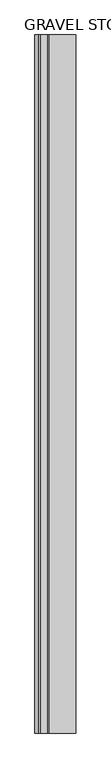
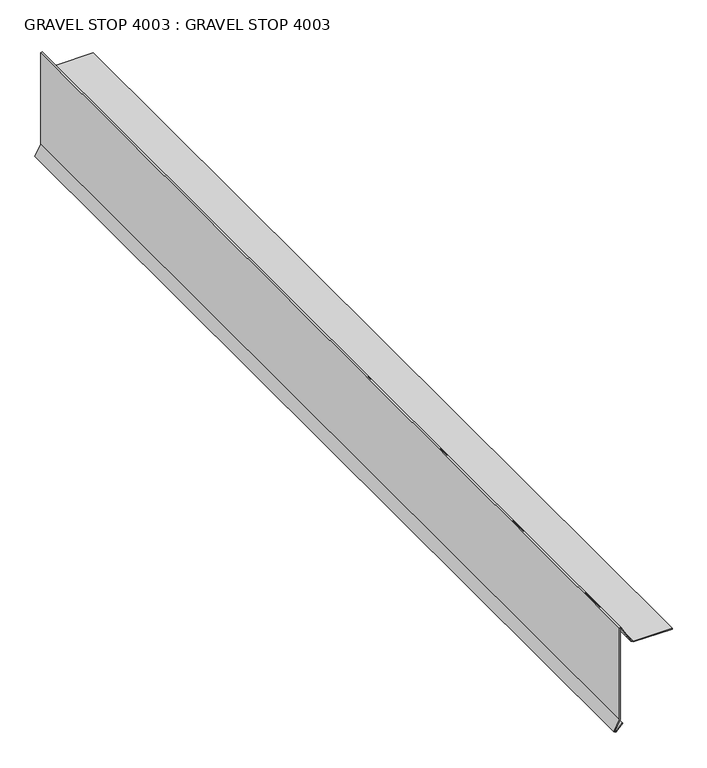
"""IFC4 building model written with IfcOpenShell, lengths in millimetres: proxy geometry, GRAVEL STOP 4003 : GRAVEL STOP 4003."""

from ifc_helpers import new_model, si_unit, frame, origin, place, context, project, spatial, polyline, outline, extrude, source, transform, mapped, element, save


def gravel_stop_4003_gravel_stop_4003_885a835c(model_context):
    return source(origin(), model_context, "Body", "SweptSolid", [
        extrude(outline(polyline([(40077.410403, -2814.9855343), (40091.8049, -2800.5910374), (40092.8027062, -2801.5888435), (40079.2807815, -2815.1107682), (40080.9054201, -2817.2404183), (40101.495749, -2805.9993985), (40293.447969, -2805.9993985), (40293.699878, -2805.0592614), (40258.5078708, -2784.7411466), (40255.9633674, -2780.3339375), (40255.9633674, -2702.4979247), (40257.3744784, -2702.4979247), (40257.3744784, -2779.9558314), (40259.5408757, -2783.7081416), (40295.3431515, -2804.3785952), (40294.5307525, -2807.4105095), (40101.8558531, -2807.4105095), (40080.5182783, -2819.0594785), (40077.410403, -2814.9855343)])), frame((0.0, -1052.8906573, 0.0), z_axis=(0.0, 1.0, 0.0), x_axis=(0.0, 0.0, 1.0)), (0.0, 0.0, 1.0), 2000.25),
    ])


if __name__ == "__main__":
    model = new_model("IFC4")
    model_context = context("Model", 3, world=origin())
    ifc_project = project(units=[si_unit("LENGTHUNIT", "METRE", prefix="MILLI")], contexts=[model_context])
    site = spatial("IfcSite", under=ifc_project)
    building = spatial("IfcBuilding", under=site)
    placement = place(None, origin())
    gravel_stop_4003_gravel_stop_4003_shape = gravel_stop_4003_gravel_stop_4003_885a835c(model_context)
    element("IfcBuildingElementProxy", 1, Name="GRAVEL STOP 4003 : GRAVEL STOP 4003", ObjectType="GRAVEL STOP 4003 : GRAVEL STOP 4003", at=placement, inside=building, context=model_context, shape_type="MappedRepresentation", body=[
        mapped(gravel_stop_4003_gravel_stop_4003_shape, transform((0.0, 0.0, 0.0), x_axis=(1.0, 0.0, 0.0), y_axis=(0.0, 1.0, 0.0), z_axis=(0.0, 0.0, 1.0))),
    ])
    save(model, "model.ifc")

# Revit data of these elements
# Type "GRAVEL STOP 4003 : GRAVEL STOP 4003"
#   NameOverride = "GRAVEL STOP"
# Element 1 (IfcBuildingElementProxy, "GRAVEL STOP 4003 : GRAVEL STOP 4003")
#   Materials on its faces: "GRAVEL STOP REQUIRED WITH GRAVEL SURFACE SYSTEMS"
# Materials
#   "GRAVEL STOP REQUIRED WITH GRAVEL SURFACE SYSTEMS": class "Unassigned", colour RGB 170 170 127, transparency 0
